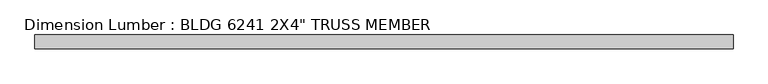
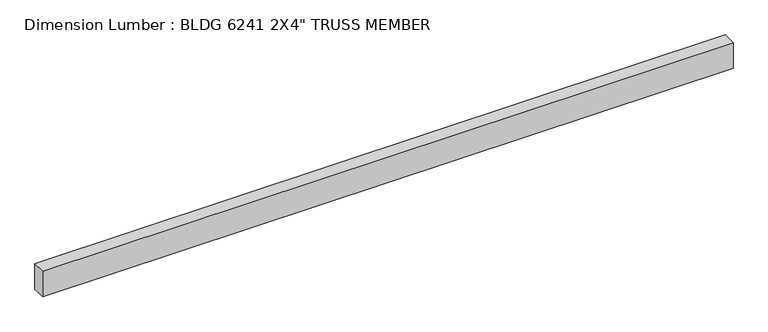
"""IFC4 building model written with IfcOpenShell, lengths in millimetres: beam geometry."""

import ifcopenshell
import ifcopenshell.guid

model = None  # the IFC model being written
_history = None  # IfcOwnerHistory: only IFC2X3 demands one
_inside = {}  # id of a spatial element -> (the spatial element, [elements in it])
_under = {}  # id of a project, library or spatial element -> (it, [spatial elements below it])
_declared = {}  # id of a project -> (the project, [libraries it declares])
_typed = {}  # id of a type object -> (the type object, [elements of that type])
_made_of = {}  # id of a material, layer set ... -> (it, [elements and type objects made of it])


def new_model(schema):
    """Start an empty IFC model of exactly this schema.

    Asked for "IFC4X3", IfcOpenShell would pick the latest addendum, in which some entities
    have other attributes; the version numbers below select the first issue.
    IFC2X3 requires an IfcOwnerHistory on every rooted entity: one is made here for all.
    """
    global model, _history
    if schema == "IFC4X3":
        model = ifcopenshell.file(schema_version=(4, 3, 0, 0))
    else:
        model = ifcopenshell.file(schema=schema)
    _inside.clear()
    _under.clear()
    _declared.clear()
    _typed.clear()
    _made_of.clear()
    _history = None
    if model.schema == "IFC2X3":
        org = make("IfcOrganization", Name="unknown")
        user = make(
            "IfcPersonAndOrganization",
            ThePerson=make("IfcPerson", FamilyName="unknown"),
            TheOrganization=org,
        )
        app = make(
            "IfcApplication",
            ApplicationDeveloper=org,
            Version="unknown",
            ApplicationFullName="unknown",
            ApplicationIdentifier="unknown",
        )
        _history = make(
            "IfcOwnerHistory",
            OwningUser=user,
            OwningApplication=app,
            ChangeAction="ADDED",
            CreationDate=0,
        )
    return model


def make(cls, **values):
    """One entity of the class cls with the attributes given. An attribute that is None is left unset."""
    return model.create_entity(
        cls, **{name: value for name, value in values.items() if value is not None}
    )


def rooted(cls, **values):
    """An entity with a GlobalId (a new one), such as an element, a storey or a relation."""
    return make(cls, GlobalId=ifcopenshell.guid.new(), OwnerHistory=_history, **values)


def si_unit(unit_type, name, prefix=None):
    """IfcSIUnit, for example si_unit("LENGTHUNIT", "METRE", prefix="MILLI")."""
    return make("IfcSIUnit", UnitType=unit_type, Prefix=prefix, Name=name)


def assignment(units):
    """IfcUnitAssignment: the units of a project."""
    return None if units is None else make("IfcUnitAssignment", Units=units)


def point(xyz):
    """IfcCartesianPoint."""
    return None if xyz is None else make("IfcCartesianPoint", Coordinates=xyz)


def direction(xyz):
    """IfcDirection."""
    return None if xyz is None else make("IfcDirection", DirectionRatios=xyz)


def frame(location, z_axis=None, x_axis=None):
    """IfcAxis2Placement3D, a coordinate frame: its origin and axes. An axis left out is left unset."""
    return make(
        "IfcAxis2Placement3D",
        Location=point(location),
        Axis=direction(z_axis),
        RefDirection=direction(x_axis),
    )


def origin():
    """The frame at (0, 0, 0) with its axes left unset."""
    return frame((0.0, 0.0, 0.0))


def place(relative_to, where):
    """IfcLocalPlacement: puts the frame where relative to a parent placement (None: the world)."""
    return make(
        "IfcLocalPlacement", PlacementRelTo=relative_to, RelativePlacement=where
    )


def context(
    kind, dimensions, precision=None, world=None, true_north=None, identifier=None
):
    """IfcGeometricRepresentationContext, for example the 3D "Model" context."""
    return make(
        "IfcGeometricRepresentationContext",
        ContextIdentifier=identifier,
        ContextType=kind,
        CoordinateSpaceDimension=dimensions,
        Precision=precision,
        WorldCoordinateSystem=world,
        TrueNorth=true_north,
    )


def project(units=None, contexts=None):
    """IfcProject with its units and contexts."""
    return rooted(
        "IfcProject",
        Name="project",
        RepresentationContexts=contexts,
        UnitsInContext=assignment(units),
    )


def spatial(cls, under=None, at=None, **own):
    """A site, building, storey or space (cls), placed at a placement, below another one or the project."""
    s = rooted(cls, ObjectPlacement=at, **own)
    if under is not None:
        _under.setdefault(under.id(), (under, []))[1].append(s)
    return s


def polyline(points):
    """IfcPolyline through the points."""
    return make("IfcPolyline", Points=[point(p) for p in points])


def outline(outer, holes=None, kind="AREA"):
    """IfcArbitraryClosedProfileDef: a profile drawn as a closed curve; with holes, ...WithVoids."""
    if holes is None:
        return make("IfcArbitraryClosedProfileDef", ProfileType=kind, OuterCurve=outer)
    return make(
        "IfcArbitraryProfileDefWithVoids",
        ProfileType=kind,
        OuterCurve=outer,
        InnerCurves=holes,
    )


def extrude(swept, where, along, depth):
    """IfcExtrudedAreaSolid: the profile swept, set in the frame where, extruded along a direction by depth."""
    return make(
        "IfcExtrudedAreaSolid",
        SweptArea=swept,
        Position=where,
        ExtrudedDirection=direction(along),
        Depth=depth,
    )


def shape(context_of_items, identifier, shape_type, items):
    """IfcShapeRepresentation: the items that make up one representation, for example the "Body"."""
    return make(
        "IfcShapeRepresentation",
        ContextOfItems=context_of_items,
        RepresentationIdentifier=identifier,
        RepresentationType=shape_type,
        Items=items,
    )


def source(mapping_origin, context_of_items, identifier, shape_type, items):
    """IfcRepresentationMap: a shape defined once, which mapped items show again and again."""
    return make(
        "IfcRepresentationMap",
        MappingOrigin=mapping_origin,
        MappedRepresentation=shape(context_of_items, identifier, shape_type, items),
    )


def transform(
    local_origin,
    x_axis=None,
    y_axis=None,
    z_axis=None,
    scale=None,
    scale2=None,
    scale3=None,
    uniform=True,
):
    """IfcCartesianTransformationOperator3D, or its non-uniform kind. x_axis, y_axis, z_axis: its Axis1, 2, 3."""
    if uniform:
        return make(
            "IfcCartesianTransformationOperator3D",
            Axis1=direction(x_axis),
            Axis2=direction(y_axis),
            LocalOrigin=point(local_origin),
            Scale=scale,
            Axis3=direction(z_axis),
        )
    return make(
        "IfcCartesianTransformationOperator3DnonUniform",
        Axis1=direction(x_axis),
        Axis2=direction(y_axis),
        LocalOrigin=point(local_origin),
        Scale=scale,
        Axis3=direction(z_axis),
        Scale2=scale2,
        Scale3=scale3,
    )


def mapped(mapping_source, mapping_target):
    """IfcMappedItem: shows the shape of a source again, moved by a transform."""
    return make(
        "IfcMappedItem", MappingSource=mapping_source, MappingTarget=mapping_target
    )


def made_of(thing, what):
    """Note that an element or type object is made of a material, layer set ...; save() writes the relation."""
    if what is not None:
        _made_of.setdefault(what.id(), (what, []))[1].append(thing)
    return thing


def element(
    cls,
    number,
    at=None,
    inside=None,
    cuts=None,
    type_object=None,
    material=None,
    context=None,
    identifier="Body",
    shape_type=None,
    held_by="IfcProductDefinitionShape",
    body=None,
    shapes=None,
    **own,
):
    """One element of the class cls, such as IfcWall. Its Tag is "e" and its number.

    at: its placement. inside: the storey or other place that contains it. cuts: it is an
    opening in that element (IfcRelVoidsElement). A single representation is given by context,
    identifier, shape_type and body (its items); several are given by shapes. held_by: the class
    of the entity that holds the representations. save() writes the other relations.
    """
    e = rooted(cls, Tag="e%d" % number, ObjectPlacement=at, **own)
    if body is not None:
        shapes = [shape(context, identifier, shape_type, body)]
    if shapes is not None:
        e.Representation = make(held_by, Representations=shapes)
    if inside is not None:
        _inside.setdefault(inside.id(), (inside, []))[1].append(e)
    if cuts is not None:
        rooted(
            "IfcRelVoidsElement", RelatingBuildingElement=cuts, RelatedOpeningElement=e
        )
    if type_object is not None:
        _typed.setdefault(type_object.id(), (type_object, []))[1].append(e)
    return made_of(e, material)


def aggregate(whole, parts):
    """IfcRelAggregates: a whole, such as a stair, and the parts it consists of."""
    return rooted("IfcRelAggregates", RelatingObject=whole, RelatedObjects=parts)


def save(model, path):
    """Write the relations noted so far, then the file.

    IfcRelAggregates (storeys below a building ...), IfcRelContainedInSpatialStructure (elements
    in a storey), IfcRelDefinesByType, IfcRelAssociatesMaterial and IfcRelDeclares: one each for
    every whole, place, type object, material and project.
    """
    for whole, parts in _under.values():
        aggregate(whole, parts)
    for where, things in _inside.values():
        rooted(
            "IfcRelContainedInSpatialStructure",
            RelatedElements=things,
            RelatingStructure=where,
        )
    for kind, things in _typed.values():
        rooted("IfcRelDefinesByType", RelatedObjects=things, RelatingType=kind)
    for what, things in _made_of.values():
        rooted("IfcRelAssociatesMaterial", RelatedObjects=things, RelatingMaterial=what)
    for by, libraries in _declared.values():
        rooted("IfcRelDeclares", RelatingContext=by, RelatedDefinitions=libraries)
    model.write(path)


def beam_d1363b41(model_context):
    return source(origin(), model_context, "Body", "SweptSolid", [
        extrude(outline(polyline([(1292.2249994, 25.4), (1292.2249994, -25.4), (-1292.2249994, -25.4), (-1292.2249994, 25.4), (1292.2249994, 25.4)])), frame((0.0, 0.0, -50.8), z_axis=(0.0, 0.0, 1.0), x_axis=(1.0, 0.0, 0.0)), (0.0, 0.0, 1.0), 101.6),
    ])


if __name__ == "__main__":
    model = new_model("IFC4")
    model_context = context("Model", 3, world=origin())
    ifc_project = project(units=[si_unit("LENGTHUNIT", "METRE", prefix="MILLI")], contexts=[model_context])
    site = spatial("IfcSite", under=ifc_project)
    building = spatial("IfcBuilding", under=site)
    placement = place(None, origin())
    beam_shape = beam_d1363b41(model_context)
    element("IfcBeam", 1, ObjectType="Dimension Lumber : BLDG 6241 2X4\" TRUSS MEMBER", at=placement, inside=building, context=model_context, shape_type="MappedRepresentation", body=[
        mapped(beam_shape, transform((0.0, 0.0, 0.0), x_axis=(1.0, 0.0, 0.0), y_axis=(0.0, 1.0, 0.0), z_axis=(0.0, 0.0, 1.0))),
    ])
    save(model, "model.ifc")

# Revit data of these elements
# Type "Dimension Lumber : BLDG 6241 2X4\" TRUSS MEMBER"
#   Assembly Code = "B10"
#   A = 0.273472 SF
#   Length [instance default] = 5' - 0"
#   b = 0' - 2"
#   d = 0' - 4"
#   Structural Material [instance default] = Softwood, Lumber
# Element 1 (IfcBeam, "Dimension Lumber : BLDG 6241 2X4\" TRUSS MEMBER")
#   Materials on its faces: "Softwood, Lumber"
# Materials
#   "Softwood, Lumber": class "Wood", colour RGB 223 192 134, transparency 0, Description = "Pinus Echinata", Cost = 0
